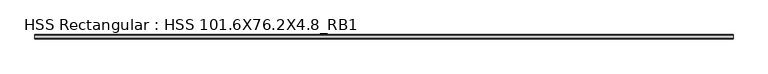
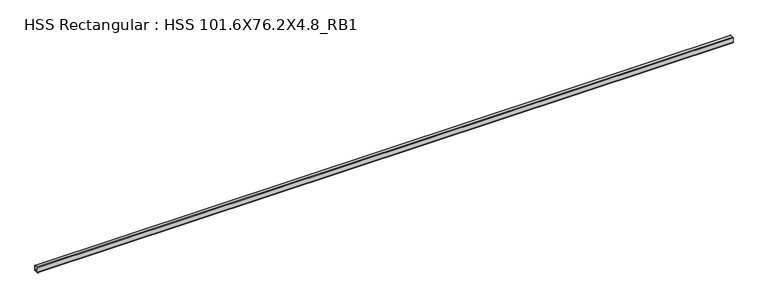
"""IFC4 building model written with IfcOpenShell, lengths in millimetres: beam geometry, HSS Rectangular : HSS 101.6X76.2X4.8_RB1."""

import ifcopenshell
import ifcopenshell.guid

model = None  # the IFC model being written
_history = None  # IfcOwnerHistory: only IFC2X3 demands one
_inside = {}  # id of a spatial element -> (the spatial element, [elements in it])
_under = {}  # id of a project, library or spatial element -> (it, [spatial elements below it])
_declared = {}  # id of a project -> (the project, [libraries it declares])
_typed = {}  # id of a type object -> (the type object, [elements of that type])
_made_of = {}  # id of a material, layer set ... -> (it, [elements and type objects made of it])


def new_model(schema):
    """Start an empty IFC model of exactly this schema.

    Asked for "IFC4X3", IfcOpenShell would pick the latest addendum, in which some entities
    have other attributes; the version numbers below select the first issue.
    IFC2X3 requires an IfcOwnerHistory on every rooted entity: one is made here for all.
    """
    global model, _history
    if schema == "IFC4X3":
        model = ifcopenshell.file(schema_version=(4, 3, 0, 0))
    else:
        model = ifcopenshell.file(schema=schema)
    _inside.clear()
    _under.clear()
    _declared.clear()
    _typed.clear()
    _made_of.clear()
    _history = None
    if model.schema == "IFC2X3":
        org = make("IfcOrganization", Name="unknown")
        user = make(
            "IfcPersonAndOrganization",
            ThePerson=make("IfcPerson", FamilyName="unknown"),
            TheOrganization=org,
        )
        app = make(
            "IfcApplication",
            ApplicationDeveloper=org,
            Version="unknown",
            ApplicationFullName="unknown",
            ApplicationIdentifier="unknown",
        )
        _history = make(
            "IfcOwnerHistory",
            OwningUser=user,
            OwningApplication=app,
            ChangeAction="ADDED",
            CreationDate=0,
        )
    return model


def make(cls, **values):
    """One entity of the class cls with the attributes given. An attribute that is None is left unset."""
    return model.create_entity(
        cls, **{name: value for name, value in values.items() if value is not None}
    )


def rooted(cls, **values):
    """An entity with a GlobalId (a new one), such as an element, a storey or a relation."""
    return make(cls, GlobalId=ifcopenshell.guid.new(), OwnerHistory=_history, **values)


def si_unit(unit_type, name, prefix=None):
    """IfcSIUnit, for example si_unit("LENGTHUNIT", "METRE", prefix="MILLI")."""
    return make("IfcSIUnit", UnitType=unit_type, Prefix=prefix, Name=name)


def assignment(units):
    """IfcUnitAssignment: the units of a project."""
    return None if units is None else make("IfcUnitAssignment", Units=units)


def point(xyz):
    """IfcCartesianPoint."""
    return None if xyz is None else make("IfcCartesianPoint", Coordinates=xyz)


def direction(xyz):
    """IfcDirection."""
    return None if xyz is None else make("IfcDirection", DirectionRatios=xyz)


def frame(location, z_axis=None, x_axis=None):
    """IfcAxis2Placement3D, a coordinate frame: its origin and axes. An axis left out is left unset."""
    return make(
        "IfcAxis2Placement3D",
        Location=point(location),
        Axis=direction(z_axis),
        RefDirection=direction(x_axis),
    )


def frame_2d(location, x_axis=None):
    """IfcAxis2Placement2D, a coordinate frame in the plane: its origin and x axis."""
    return make(
        "IfcAxis2Placement2D", Location=point(location), RefDirection=direction(x_axis)
    )


def origin():
    """The frame at (0, 0, 0) with its axes left unset."""
    return frame((0.0, 0.0, 0.0))


def place(relative_to, where):
    """IfcLocalPlacement: puts the frame where relative to a parent placement (None: the world)."""
    return make(
        "IfcLocalPlacement", PlacementRelTo=relative_to, RelativePlacement=where
    )


def context(
    kind, dimensions, precision=None, world=None, true_north=None, identifier=None
):
    """IfcGeometricRepresentationContext, for example the 3D "Model" context."""
    return make(
        "IfcGeometricRepresentationContext",
        ContextIdentifier=identifier,
        ContextType=kind,
        CoordinateSpaceDimension=dimensions,
        Precision=precision,
        WorldCoordinateSystem=world,
        TrueNorth=true_north,
    )


def project(units=None, contexts=None):
    """IfcProject with its units and contexts."""
    return rooted(
        "IfcProject",
        Name="project",
        RepresentationContexts=contexts,
        UnitsInContext=assignment(units),
    )


def spatial(cls, under=None, at=None, **own):
    """A site, building, storey or space (cls), placed at a placement, below another one or the project."""
    s = rooted(cls, ObjectPlacement=at, **own)
    if under is not None:
        _under.setdefault(under.id(), (under, []))[1].append(s)
    return s


def polyline(points):
    """IfcPolyline through the points."""
    return make("IfcPolyline", Points=[point(p) for p in points])


def circle_curve(where, radius):
    """IfcCircle in the frame where."""
    return make("IfcCircle", Position=where, Radius=radius)


def trimmed(basis, trim1, trim2, sense, master):
    """IfcTrimmedCurve: the piece of a basis curve between two trims."""
    return make(
        "IfcTrimmedCurve",
        BasisCurve=basis,
        Trim1=trim1,
        Trim2=trim2,
        SenseAgreement=sense,
        MasterRepresentation=master,
    )


def segment(curve, same_sense, transition):
    """IfcCompositeCurveSegment."""
    return make(
        "IfcCompositeCurveSegment",
        Transition=transition,
        SameSense=same_sense,
        ParentCurve=curve,
    )


def composite_curve(segments, self_intersect=None):
    """IfcCompositeCurve: segments joined end to end."""
    return make("IfcCompositeCurve", Segments=segments, SelfIntersect=self_intersect)


def outline(outer, holes=None, kind="AREA"):
    """IfcArbitraryClosedProfileDef: a profile drawn as a closed curve; with holes, ...WithVoids."""
    if holes is None:
        return make("IfcArbitraryClosedProfileDef", ProfileType=kind, OuterCurve=outer)
    return make(
        "IfcArbitraryProfileDefWithVoids",
        ProfileType=kind,
        OuterCurve=outer,
        InnerCurves=holes,
    )


def extrude(swept, where, along, depth):
    """IfcExtrudedAreaSolid: the profile swept, set in the frame where, extruded along a direction by depth."""
    return make(
        "IfcExtrudedAreaSolid",
        SweptArea=swept,
        Position=where,
        ExtrudedDirection=direction(along),
        Depth=depth,
    )


def shape(context_of_items, identifier, shape_type, items):
    """IfcShapeRepresentation: the items that make up one representation, for example the "Body"."""
    return make(
        "IfcShapeRepresentation",
        ContextOfItems=context_of_items,
        RepresentationIdentifier=identifier,
        RepresentationType=shape_type,
        Items=items,
    )


def source(mapping_origin, context_of_items, identifier, shape_type, items):
    """IfcRepresentationMap: a shape defined once, which mapped items show again and again."""
    return make(
        "IfcRepresentationMap",
        MappingOrigin=mapping_origin,
        MappedRepresentation=shape(context_of_items, identifier, shape_type, items),
    )


def transform(
    local_origin,
    x_axis=None,
    y_axis=None,
    z_axis=None,
    scale=None,
    scale2=None,
    scale3=None,
    uniform=True,
):
    """IfcCartesianTransformationOperator3D, or its non-uniform kind. x_axis, y_axis, z_axis: its Axis1, 2, 3."""
    if uniform:
        return make(
            "IfcCartesianTransformationOperator3D",
            Axis1=direction(x_axis),
            Axis2=direction(y_axis),
            LocalOrigin=point(local_origin),
            Scale=scale,
            Axis3=direction(z_axis),
        )
    return make(
        "IfcCartesianTransformationOperator3DnonUniform",
        Axis1=direction(x_axis),
        Axis2=direction(y_axis),
        LocalOrigin=point(local_origin),
        Scale=scale,
        Axis3=direction(z_axis),
        Scale2=scale2,
        Scale3=scale3,
    )


def mapped(mapping_source, mapping_target):
    """IfcMappedItem: shows the shape of a source again, moved by a transform."""
    return make(
        "IfcMappedItem", MappingSource=mapping_source, MappingTarget=mapping_target
    )


def made_of(thing, what):
    """Note that an element or type object is made of a material, layer set ...; save() writes the relation."""
    if what is not None:
        _made_of.setdefault(what.id(), (what, []))[1].append(thing)
    return thing


def element(
    cls,
    number,
    at=None,
    inside=None,
    cuts=None,
    type_object=None,
    material=None,
    context=None,
    identifier="Body",
    shape_type=None,
    held_by="IfcProductDefinitionShape",
    body=None,
    shapes=None,
    **own,
):
    """One element of the class cls, such as IfcWall. Its Tag is "e" and its number.

    at: its placement. inside: the storey or other place that contains it. cuts: it is an
    opening in that element (IfcRelVoidsElement). A single representation is given by context,
    identifier, shape_type and body (its items); several are given by shapes. held_by: the class
    of the entity that holds the representations. save() writes the other relations.
    """
    e = rooted(cls, Tag="e%d" % number, ObjectPlacement=at, **own)
    if body is not None:
        shapes = [shape(context, identifier, shape_type, body)]
    if shapes is not None:
        e.Representation = make(held_by, Representations=shapes)
    if inside is not None:
        _inside.setdefault(inside.id(), (inside, []))[1].append(e)
    if cuts is not None:
        rooted(
            "IfcRelVoidsElement", RelatingBuildingElement=cuts, RelatedOpeningElement=e
        )
    if type_object is not None:
        _typed.setdefault(type_object.id(), (type_object, []))[1].append(e)
    return made_of(e, material)


def aggregate(whole, parts):
    """IfcRelAggregates: a whole, such as a stair, and the parts it consists of."""
    return rooted("IfcRelAggregates", RelatingObject=whole, RelatedObjects=parts)


def save(model, path):
    """Write the relations noted so far, then the file.

    IfcRelAggregates (storeys below a building ...), IfcRelContainedInSpatialStructure (elements
    in a storey), IfcRelDefinesByType, IfcRelAssociatesMaterial and IfcRelDeclares: one each for
    every whole, place, type object, material and project.
    """
    for whole, parts in _under.values():
        aggregate(whole, parts)
    for where, things in _inside.values():
        rooted(
            "IfcRelContainedInSpatialStructure",
            RelatedElements=things,
            RelatingStructure=where,
        )
    for kind, things in _typed.values():
        rooted("IfcRelDefinesByType", RelatedObjects=things, RelatingType=kind)
    for what, things in _made_of.values():
        rooted("IfcRelAssociatesMaterial", RelatedObjects=things, RelatingMaterial=what)
    for by, libraries in _declared.values():
        rooted("IfcRelDeclares", RelatingContext=by, RelatedDefinitions=libraries)
    model.write(path)


def hss_rectangular_hss_101_6x76_2x4_8_rb1_e15d674e(model_context):
    return source(origin(), model_context, "Body", "SweptSolid", [
        extrude(outline(composite_curve([segment(trimmed(circle_curve(frame_2d((-28.575, 41.275)), 9.525), [point((-38.1, 41.275))], [point((-28.575, 50.8))], False, "CARTESIAN"), True, "CONTINUOUS"), segment(polyline([(-28.575, 50.8), (28.575, 50.8)]), True, "CONTINUOUS"), segment(trimmed(circle_curve(frame_2d((28.575, 41.275)), 9.525), [point((28.575, 50.8))], [point((38.1, 41.275))], False, "CARTESIAN"), True, "CONTINUOUS"), segment(polyline([(38.1, 41.275), (38.1, -41.275)]), True, "CONTINUOUS"), segment(trimmed(circle_curve(frame_2d((28.575, -41.275)), 9.525), [point((38.1, -41.275))], [point((28.575, -50.8))], False, "CARTESIAN"), True, "CONTINUOUS"), segment(polyline([(28.575, -50.8), (-28.575, -50.8)]), True, "CONTINUOUS"), segment(trimmed(circle_curve(frame_2d((-28.575, -41.275)), 9.525), [point((-28.575, -50.8))], [point((-38.1, -41.275))], False, "CARTESIAN"), True, "CONTINUOUS"), segment(polyline([(-38.1, -41.275), (-38.1, 41.275)]), True, "CONTINUOUS")], self_intersect=False), holes=[composite_curve([segment(polyline([(28.575, 46.0375), (-28.575, 46.0375)]), True, "CONTINUOUS"), segment(trimmed(circle_curve(frame_2d((-28.575, 41.275)), 4.7625), [point((-28.575, 46.0375))], [point((-33.3375, 41.275))], True, "CARTESIAN"), True, "CONTINUOUS"), segment(polyline([(-33.3375, 41.275), (-33.3375, -41.275)]), True, "CONTINUOUS"), segment(trimmed(circle_curve(frame_2d((-28.575, -41.275)), 4.7625), [point((-33.3375, -41.275))], [point((-28.575, -46.0375))], True, "CARTESIAN"), True, "CONTINUOUS"), segment(polyline([(-28.575, -46.0375), (28.575, -46.0375)]), True, "CONTINUOUS"), segment(trimmed(circle_curve(frame_2d((28.575, -41.275)), 4.7625), [point((28.575, -46.0375))], [point((33.3375, -41.275))], True, "CARTESIAN"), True, "CONTINUOUS"), segment(polyline([(33.3375, -41.275), (33.3375, 41.275)]), True, "CONTINUOUS"), segment(trimmed(circle_curve(frame_2d((28.575, 41.275)), 4.7625), [point((33.3375, 41.275))], [point((28.575, 46.0375))], True, "CARTESIAN"), True, "CONTINUOUS")], self_intersect=False)]), frame((-7490.0, 0.0, 0.0), z_axis=(1.0, 0.0, 0.0), x_axis=(0.0, 1.0, 0.0)), (0.0, 0.0, 1.0), 12023.3951902),
    ])


if __name__ == "__main__":
    model = new_model("IFC4")
    model_context = context("Model", 3, world=origin())
    ifc_project = project(units=[si_unit("LENGTHUNIT", "METRE", prefix="MILLI")], contexts=[model_context])
    site = spatial("IfcSite", under=ifc_project)
    building = spatial("IfcBuilding", under=site)
    placement = place(None, origin())
    hss_rectangular_hss_101_6x76_2x4_8_rb1_shape = hss_rectangular_hss_101_6x76_2x4_8_rb1_e15d674e(model_context)
    element("IfcBeam", 1, ObjectType="HSS Rectangular : HSS 101.6X76.2X4.8_RB1", at=placement, inside=building, context=model_context, shape_type="MappedRepresentation", body=[
        mapped(hss_rectangular_hss_101_6x76_2x4_8_rb1_shape, transform((0.0, 0.0, 0.0), x_axis=(1.0, 0.0, 0.0), y_axis=(0.0, 1.0, 0.0), z_axis=(0.0, 0.0, 1.0))),
    ])
    save(model, "model.ifc")

# Revit data of these elements
# Type "HSS Rectangular : HSS 101.6X76.2X4.8_RB1"
#   Section Name Key = "HSS 4X3X3/16"
#   Assembly Code = "B10"
#   Width = 7.62 cm
#   Wall Nominal Thickness = 0.4763 cm
#   Wall Design Thickness = 0.442 cm
#   Torsional Moment of Inertia = 260.561 cm⁴
#   Torsional Modulus = 61.2876 cm³
#   Section Area = 14.4516 cm²
#   Plastic Modulus weak axis = 40.3122 cm³
#   Plastic Modulus strong axis = 49.1612 cm³
#   Perimeter = 0.881482 m²/m
#   Outer Fillet = 0.9525 cm
#   Nominal Weight = 12.1285 kgf/m
#   Moment of Inertia weak axis = 131.529 cm⁴
#   Moment of Inertia strong axis = 205.202 cm⁴
#   Inner Fillet = 0.4763 cm
#   Height = 10.16 cm
#   Elastic Modulus weak axis = 34.4128 cm³
#   Elastic Modulus strong axis = 40.476 cm³
#   Centroid Vertical = 5.08 cm
#   Centroid Horizontal = 3.81 cm
#   Length [instance default] = 1524 mm
#   Structural Material [instance default] = Steel ASTM A500, Grade B, Rectangular and Square
#   Principal Axes Angle = 0
# Element 1 (IfcBeam, "HSS Rectangular : HSS 101.6X76.2X4.8_RB1")
#   Structural Material = Steel ASTM A992
#   Materials on its faces: "Steel ASTM A992"
# Materials
#   "Steel ASTM A500, Grade B, Rectangular and Square": class "Metal", colour RGB 199 199 199, transparency 0, Description = "Carbon steel", Cost = 0
#   "Steel ASTM A992": class "Metal", colour RGB 199 199 199, transparency 0, Description = "Structural steel 50ksi", Cost = 0
